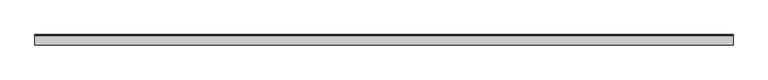
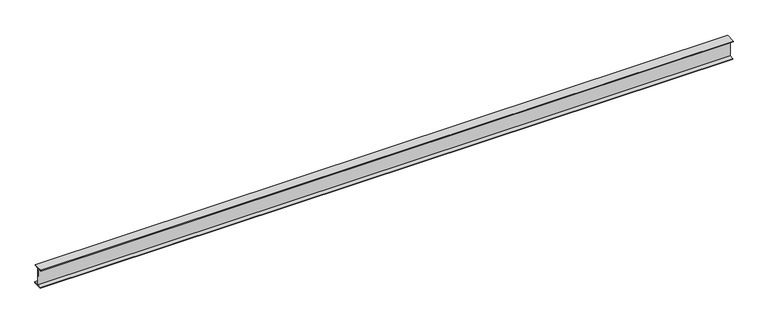
"""IFC4 building model written with IfcOpenShell, lengths in millimetres: proxy geometry, Generic Models 7:Generic Models 1:8:Generic Models 1:8 : Generic Models 7:Generic Models 1:337419:25 : Generic Models 7:Generic Models 1:8:Generic Models 1:8 : Generic Models 7:Generic Models 1:337419:315935."""

from ifc_helpers import new_model, si_unit, frame, origin, place, context, project, spatial, polyline, outline, extrude, source, transform, mapped, element, save


def generic_models_9ca1a4a2(model_context):
    return source(origin(), model_context, "Body", "SweptSolid", [
        extrude(outline(polyline([(-564811.1638405, 8910.9108708), (-564811.4969265, 8918.9049345), (-564709.7312265, 8923.145172), (-564709.3981405, 8915.1511083), (-564757.1721879, 8913.160523), (-564749.2627175, 8723.3332321), (-564701.48867, 8725.3238175), (-564701.155584, 8717.3297537), (-564802.921284, 8713.0895162), (-564803.25437, 8721.08358), (-564755.4803226, 8723.0741653), (-564763.389793, 8912.9014561), (-564811.1638405, 8910.9108708)])), frame((588867.6367242, 0.0, 0.0), z_axis=(1.0, 0.0, 0.0), x_axis=(0.0, 1.0, 0.0)), (0.0, 0.0, 1.0), 7315.2),
    ])


if __name__ == "__main__":
    model = new_model("IFC4")
    model_context = context("Model", 3, world=origin())
    ifc_project = project(units=[si_unit("LENGTHUNIT", "METRE", prefix="MILLI")], contexts=[model_context])
    site = spatial("IfcSite", under=ifc_project)
    building = spatial("IfcBuilding", under=site)
    placement = place(None, origin())
    generic_models_shape = generic_models_9ca1a4a2(model_context)
    element("IfcBuildingElementProxy", 1, Name="Generic Models 7:Generic Models 1:8:Generic Models 1:8 : Generic Models 7:Generic Models 1:337419:25 : Generic Models 7:Generic Models 1:8:Generic Models 1:8 : Generic Models 7:Generic Models 1:337419:315935", ObjectType="Generic Models 7:Generic Models 1:8:Generic Models 1:8 : Generic Models 7:Generic Models 1:337419:25 : Generic Models 7:Generic Models 1:8:Generic Models 1:8 : Generic Models 7:Generic Models 1:337419:315935", at=placement, inside=building, context=model_context, shape_type="MappedRepresentation", body=[
        mapped(generic_models_shape, transform((0.0, 0.0, 0.0), x_axis=(1.0, 0.0, 0.0), y_axis=(0.0, 1.0, 0.0), z_axis=(0.0, 0.0, 1.0))),
    ])
    save(model, "model.ifc")

# Revit data of these elements
# Type "Generic Models 7:Generic Models 1:8:Generic Models 1:8 : Generic Models 7:Generic Models 1:337419:25 : Generic Models 7:Generic Models 1:8:Generic Models 1:8 : Generic Models 7:Generic Models 1:337419:315935"
#   NameOverride = "Generic Models 7:Generic Models 1:8:Generic Models 1:8 : Generic Models 7:Generic Models 1:337419:315935"
#   ObjectTypeOverride = "Generic Models 1:8 : Generic Models 7:Generic Models 1:337419"
#   Reference = "Generic Models 1"
#   Tag = "315935"
# Element 1 (IfcBuildingElementProxy, "Generic Models 7:Generic Models 1:8:Generic Models 1:8 : Generic Models 7:Generic Models 1:337419:25 : Generic Models 7:Generic Models 1:8:Generic Models 1:8 : Generic Models 7:Generic Models 1:337419:315935")
#   Materials on its faces: "STRUCTURAL STEEL - SEE STRUCT. DWGS"
# Materials
#   "STRUCTURAL STEEL - SEE STRUCT. DWGS": class "Metal", colour RGB 189 187 185, transparency 0, Description = "Structural steel 50ksi", Cost = 0
